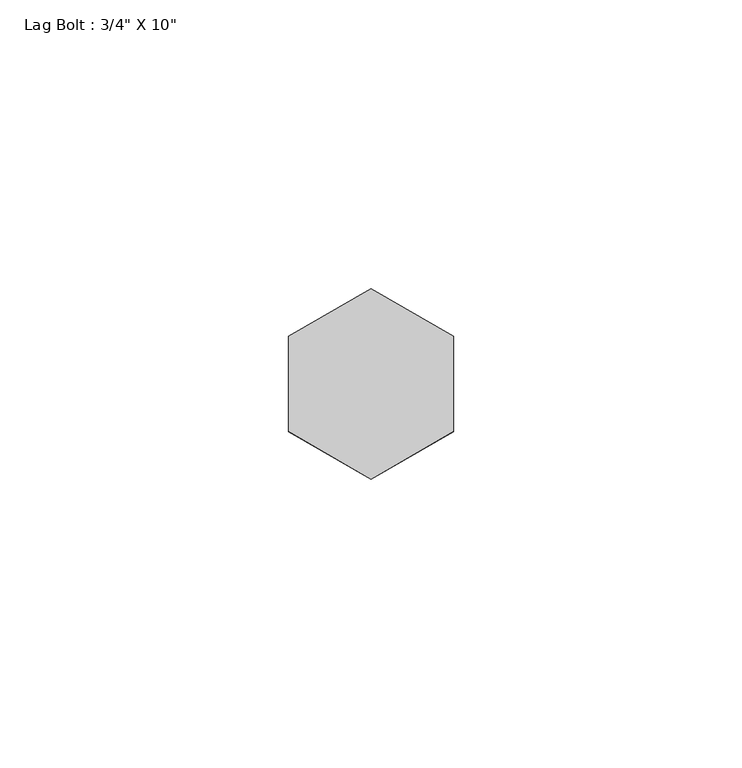
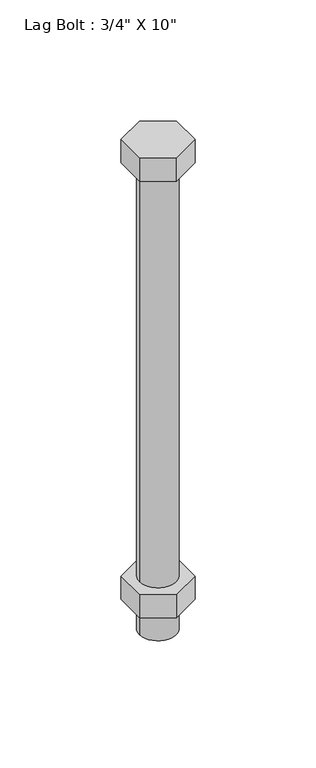
"""IFC4 building model written with IfcOpenShell, lengths in millimetres: proxy geometry."""

from ifc_helpers import new_model, si_unit, point, frame, origin, origin_with_axes, origin_2d, place, context, project, spatial, polyline, circle_curve, trimmed, segment, composite_curve, outline, extrude, source, transform, mapped, element, save


def proxy_4fadfd69(model_context):
    return source(origin(), model_context, "Body", "SweptSolid", [
        extrude(outline(polyline([(-14.2875, 8.248892), (0.0, 16.4977839), (14.2875, 8.248892), (14.2875, -8.248892), (0.0, -16.4977839), (-14.2875, -8.248892), (-14.2875, 8.248892)])), frame((0.0, 0.0, -238.125), z_axis=(0.0, 0.0, 1.0), x_axis=(1.0, 0.0, 0.0)), (0.0, 0.0, 1.0), 12.7),
        extrude(outline(polyline([(-14.2875, -8.248892), (-14.2875, 8.248892), (0.0, 16.4977839), (14.2875, 8.248892), (14.2875, -8.248892), (0.0, -16.4977839), (-14.2875, -8.248892)])), origin_with_axes(), (0.0, 0.0, 1.0), 12.7),
        extrude(outline(composite_curve([segment(trimmed(circle_curve(origin_2d(), 9.525), [point((-9.525, 0.0))], [point((9.525, 0.0))], False, "CARTESIAN"), True, "CONTINUOUS"), segment(trimmed(circle_curve(origin_2d(), 9.525), [point((9.525, 0.0))], [point((-9.525, 0.0))], False, "CARTESIAN"), True, "CONTINUOUS")], self_intersect=False)), frame((0.0, 0.0, -254.0), z_axis=(0.0, 0.0, 1.0), x_axis=(1.0, 0.0, 0.0)), (0.0, 0.0, 1.0), 254.0),
    ])


if __name__ == "__main__":
    model = new_model("IFC4")
    model_context = context("Model", 3, world=origin())
    ifc_project = project(units=[si_unit("LENGTHUNIT", "METRE", prefix="MILLI")], contexts=[model_context])
    site = spatial("IfcSite", under=ifc_project)
    building = spatial("IfcBuilding", under=site)
    placement = place(None, origin())
    proxy_shape = proxy_4fadfd69(model_context)
    element("IfcBuildingElementProxy", 1, Name="Lag Bolt : 3/4\" X 10\"", ObjectType="Lag Bolt : 3/4\" X 10\"", at=placement, inside=building, context=model_context, shape_type="MappedRepresentation", body=[
        mapped(proxy_shape, transform((0.0, 0.0, 0.0), x_axis=(1.0, 0.0, 0.0), y_axis=(0.0, 1.0, 0.0), z_axis=(0.0, 0.0, 1.0))),
    ])
    save(model, "model.ifc")

# Revit data of these elements
# Type "Lag Bolt : 3/4\" X 10\""
#   Thickness_of_Substrate [instance default] = 0' - 1"
#   Side = 0' - 0.65039"
#   Radius = 0' - 0 3/8"
#   Length = 0' - 10"
#   Head Size = 0' - 1 1/8"
#   Head Radius = 0' - 0 9/16"
#   Head Height = 0' - 0 1/2"
#   Diameter = 0' - 0 3/4"
#   Default Elevation = 4' - 0"
#   Nut_Visibility [instance default] = yes
#   Bolt Material (Size) [instance default] = 5/8" GALV. ANCHOR BOLT @ 24" O.C. (6" MIN. EMBEDMENT)
# Element 1 (IfcBuildingElementProxy, "Lag Bolt : 3/4\" X 10\"")
#   Thickness_of_Substrate = 0' - 8 7/8"
#   Bolt Material (Size) = (3) 3/4" THU BOLT
#   Materials on its faces: "(3) 3/4\" THU BOLT"
# Materials
#   "5/8\" GALV. ANCHOR BOLT @ 24\" O.C. (6\" MIN. EMBEDMENT)": class "Generic", colour RGB 120 120 120, transparency 0, Cost = 0
#   "(3) 3/4\" THU BOLT": class "Generic", colour RGB 120 120 120, transparency 0, Cost = 0
